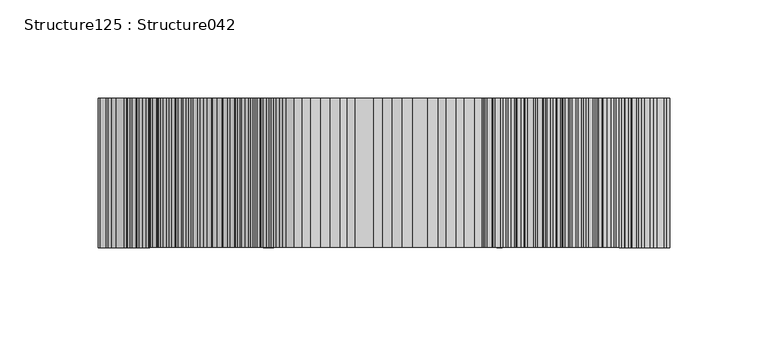
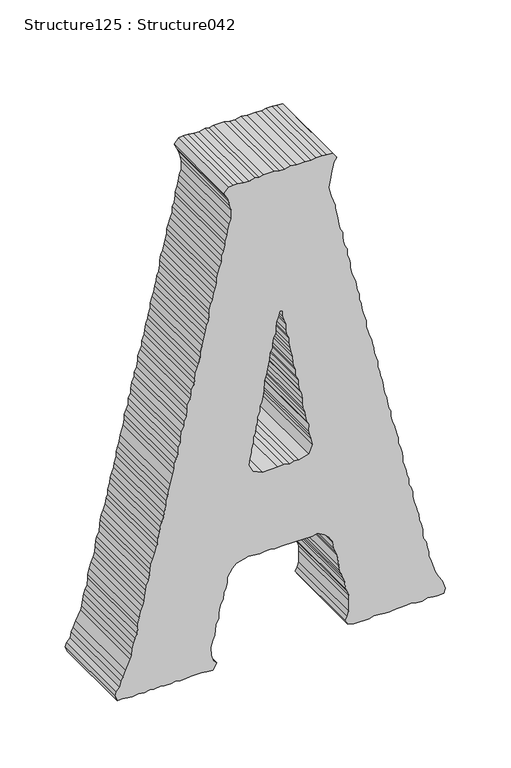
"""IFC4 building model written with IfcOpenShell, lengths in millimetres: proxy geometry, Structure125 : Structure042."""

from ifc_helpers import new_model, si_unit, frame, origin, place, context, project, spatial, polyline, outline, extrude, source, transform, mapped, element, save


def structure125_structure042_6af9a522(model_context):
    return source(origin(), model_context, "Body", "SweptSolid", [
        extrude(outline(polyline([(3818.8310229, -41243.193379), (3814.7296538, -41243.193379), (3811.2043377, -41244.3743679), (3805.9476534, -41246.6914168), (3801.8462843, -41246.6914168), (3795.960595, -41247.2931435), (3791.8865042, -41249.6326569), (3787.7867397, -41249.6326569), (3783.0868532, -41251.9962393), (3777.8285642, -41252.5755015), (3773.11905, -41252.5755015), (3769.6274306, -41254.9150149), (3763.759392, -41254.9150149), (3759.6596275, -41256.675266), (3755.559863, -41258.4371217), (3750.8583719, -41258.4371217), (3746.1745313, -41259.5956462), (3737.400554, -41261.9351595), (3732.1149867, -41263.1161484), (3727.4311462, -41264.2746729), (3723.3313817, -41265.4572664), (3718.6571688, -41265.4572664), (3713.3555556, -41267.2175175), (3709.2718371, -41267.8192442), (3704.5879966, -41269.5570309), (3701.0723082, -41270.7155553), (3695.786741, -41271.317282), (3690.512406, -41273.0791377), (3685.8285655, -41273.0791377), (3682.8857208, -41274.2601267), (3677.6274319, -41275.4186511), (3672.9435914, -41277.1789022), (3668.8261762, -41278.9391534), (3664.1423357, -41279.5184156), (3660.0682449, -41280.0992824), (3654.1841602, -41280.7010091), (3650.1004418, -41283.0405225), (3645.9830266, -41283.6422491), (3641.2991861, -41284.1990469), (3636.0408972, -41284.7783091), (3631.915459, -41285.959298), (3627.8397636, -41287.7211538), (3622.555801, -41289.4814049), (3617.2718384, -41290.6623938), (3613.772196, -41290.6623938), (3607.8961343, -41291.241656), (3604.3964919, -41293.0019072), (3600.2967274, -41294.1604316), (3595.5872132, -41295.3430251), (3589.7544759, -41295.9222873), (3586.2115092, -41297.1032763), (3577.4535778, -41301.2030407), (3572.1423369, -41303.5441587), (3568.6426945, -41305.3044098), (3563.366755, -41306.4629343), (3560.441561, -41309.4041743), (3556.3417965, -41310.5867678), (3551.6675836, -41308.8024476), (3551.6675836, -41304.1458854), (3551.0658569, -41299.4427896), (3550.4833855, -41295.3430251), (3551.6675836, -41290.0831316), (3550.4833855, -41284.7783091), (3551.6675836, -41280.0992824), (3551.0658569, -41276.5771755), (3551.6675836, -41270.7155553), (3551.0658569, -41267.2175175), (3551.0658569, -41261.3783618), (3551.6675836, -41257.2545282), (3551.0658569, -41253.1547637), (3551.0658569, -41248.4516679), (3551.6675836, -41243.7726412), (3551.6675836, -41234.4113786), (3551.0658569, -41229.7323519), (3550.4833855, -41224.4275294), (3556.3417965, -41220.9294916), (3559.2669905, -41223.8482672), (3565.1254015, -41225.6085183), (3572.7440636, -41226.1877806), (3578.6104977, -41224.4275294), (3582.7102621, -41222.6897428), (3587.3860796, -41222.1104805), (3592.0955938, -41221.5087539), (3596.7698067, -41219.1676359), (3601.4536473, -41219.1676359), (3604.9709403, -41218.5883737), (3610.2292293, -41217.4073848), (3613.772196, -41215.0678714), (3619.6145609, -41214.4886092), (3622.555801, -41212.7267535), (3627.8397636, -41211.5457645), (3633.0980525, -41211.5457645), (3639.5405396, -41206.8667378), (3643.0578326, -41203.344631), (3644.8245022, -41196.3244863), (3645.9830266, -41192.803984), (3645.4262289, -41186.9423638), (3644.8245022, -41182.8409947), (3645.4262289, -41178.161968), (3645.9830266, -41173.4588722), (3644.8245022, -41169.3815722), (3645.4262289, -41164.0767497), (3645.4262289, -41151.7967115), (3644.8245022, -41145.9350913), (3644.8245022, -41136.5529688), (3645.9830266, -41131.8739421), (3642.4833842, -41125.4330597), (3638.9580681, -41121.3092261), (3633.0980525, -41118.412915), (3627.2396415, -41117.2319261), (3622.555801, -41115.4700704), (3619.6145609, -41114.2890815), (3609.0723094, -41113.1080925), (3604.3964919, -41111.9271036), (3600.2967274, -41110.7910437), (3596.1953583, -41109.0291879), (3592.0955938, -41107.848199), (3586.2115092, -41107.2689368), (3582.7102621, -41105.4862212), (3578.6104977, -41104.3276967), (3573.9266571, -41104.3276967), (3563.9412034, -41104.3276967), (3559.2669905, -41105.4862212), (3555.7416744, -41107.2689368), (3551.6675836, -41104.906959), (3550.4833855, -41099.6470654), (3550.4833855, -41086.1635739), (3551.6675836, -41082.0638094), (3551.0658569, -41076.7814514), (3550.4833855, -41072.1024247), (3550.4833855, -41068.0010556), (3551.0658569, -41062.1394353), (3551.0658569, -41058.0621353), (3551.6675836, -41053.3590395), (3551.6675836, -41049.2576705), (3550.4833855, -41044.5561793), (3550.4833855, -41039.2962857), (3551.6675836, -41034.6156544), (3551.0658569, -41029.3124366), (3550.4833855, -41025.8127942), (3551.0658569, -41019.9736384), (3555.1848766, -41018.7926495), (3560.441561, -41020.5545052), (3563.366755, -41021.7130297), (3568.6426945, -41025.2335319), (3572.1423369, -41026.9937831), (3576.2693797, -41028.7556388), (3586.2115092, -41031.6744144), (3590.3289243, -41033.4346655), (3594.4286888, -41033.4346655), (3599.1125293, -41034.6156544), (3604.3964919, -41035.7757835), (3608.4705827, -41038.1152968), (3612.5976255, -41038.6945591), (3617.2718384, -41038.6945591), (3622.555801, -41039.875548), (3627.2396415, -41041.6357991), (3632.5155811, -41042.2375258), (3636.0408972, -41043.3976548), (3640.114988, -41044.5561793), (3645.4262289, -41046.3164304), (3650.6845178, -41047.4974193), (3655.3587307, -41047.4974193), (3659.4584952, -41048.6784082), (3663.5598643, -41051.0195262), (3668.8261762, -41051.0195262), (3673.5276674, -41052.7573129), (3677.0449605, -41053.3590395), (3682.8857208, -41055.1192907), (3686.4030139, -41056.2778151), (3691.0868544, -41056.2778151), (3695.2122926, -41056.8795418), (3699.8881101, -41058.0621353), (3705.7545441, -41060.3791842), (3710.4560353, -41060.3791842), (3714.5301261, -41061.5601731), (3718.0554422, -41062.7186976), (3723.3313817, -41063.8996865), (3727.4311462, -41065.6615422), (3732.7167134, -41066.8200667), (3737.9750024, -41066.8200667), (3740.9162424, -41068.5803178), (3745.6000829, -41069.7613067), (3751.4424479, -41070.3405689), (3756.1423345, -41072.1024247), (3759.6596275, -41073.2834136), (3764.3611187, -41073.8402113), (3769.0176809, -41074.441938), (3774.3032481, -41076.2021891), (3777.8285642, -41076.7814514), (3783.0868532, -41078.5417025), (3788.3611881, -41078.5417025), (3791.8865042, -41079.724296), (3797.1463977, -41081.4620827), (3801.8462843, -41082.0638094), (3806.5317294, -41083.2223338), (3810.0474179, -41083.8240605), (3815.3313805, -41086.1635739), (3820.015221, -41087.3461674), (3824.1149855, -41088.5271563), (3829.374879, -41088.5271563), (3837.6000817, -41091.4459319), (3842.8583706, -41092.6044563), (3846.9757858, -41093.206183), (3851.6612309, -41094.9680387), (3856.9179152, -41094.9680387), (3861.0192843, -41096.7058254), (3866.3032469, -41097.2850876), (3869.8189354, -41097.8868143), (3873.9203044, -41099.6470654), (3878.5784713, -41101.4073166), (3883.8881076, -41102.5899101), (3888.5623205, -41102.5899101), (3892.6636896, -41103.7484345), (3897.3475301, -41105.4862212), (3902.6314927, -41105.4862212), (3906.1487857, -41107.848199), (3910.8310217, -41109.0291879), (3916.0909152, -41109.6100547), (3919.6066036, -41109.6100547), (3924.2888396, -41111.9271036), (3928.9919353, -41113.1080925), (3934.2758979, -41113.7098192), (3938.9517154, -41114.8683437), (3944.235678, -41116.0493326), (3947.1496398, -41116.0493326), (3956.5349715, -41119.548975), (3961.794865, -41120.7299639), (3965.8930249, -41121.9109528), (3974.7055128, -41120.1507017), (3979.9621971, -41118.9697128), (3983.4794902, -41118.412915), (3987.5792547, -41117.2319261), (3991.6806238, -41114.8683437), (3996.390138, -41118.412915), (3996.9645864, -41123.6712039), (3997.5486624, -41127.7501086), (3997.5486624, -41133.054931), (3996.390138, -41137.1322311), (3996.9645864, -41142.4145891), (3996.9645864, -41150.0139959), (3997.5486624, -41155.3188184), (3996.390138, -41160.5771073), (3996.390138, -41165.2577387), (3997.5486624, -41169.9608344), (3997.5486624, -41179.3204925), (3996.9645864, -41183.4218615), (3997.5486624, -41186.9423638), (3996.390138, -41192.2247218), (3996.390138, -41196.9037485), (3997.5486624, -41202.1636421), (3997.5486624, -41206.2874756), (3996.9645864, -41210.3647756), (3992.2614906, -41214.4886092), (3987.5792547, -41212.1474912), (3984.0635662, -41210.3647756), (3979.3781211, -41209.2062512), (3974.7055128, -41208.0477267), (3966.5043792, -41208.0477267), (3962.3757319, -41209.7855134), (3957.1190475, -41210.9665023), (3952.435207, -41211.5457645), (3947.7337158, -41213.3076203), (3944.235678, -41213.3076203), (3938.3499888, -41214.4886092), (3934.8503464, -41216.2488603), (3929.5904528, -41216.2488603), (3924.8905662, -41217.986647), (3919.6066036, -41219.7468981), (3915.5068392, -41220.9294916), (3910.8310217, -41220.9294916), (3906.1487857, -41222.1104805), (3902.6314927, -41223.2914695), (3896.763454, -41224.4275294), (3893.822214, -41226.1877806), (3888.5623205, -41227.3687695), (3884.4609514, -41227.3687695), (3878.5784713, -41227.9704962), (3875.0772243, -41229.7323519), (3870.4030114, -41230.3116141), (3866.3032469, -41231.4701386), (3861.0192843, -41232.628663), (3856.9179152, -41233.8096519), (3851.6612309, -41235.5715077), (3846.9757858, -41235.5715077), (3841.6741725, -41237.3317588), (3838.1761347, -41237.9334855), (3833.4730389, -41239.6712721), (3828.2163546, -41240.2505344), (3824.1149855, -41240.8522611), (3818.8310229, -41243.193379)]), holes=[polyline([(3720.4158154, -41180.5014814), (3723.9154578, -41188.7026149), (3730.9323932, -41192.2247218), (3736.7988273, -41191.0437329), (3741.5003184, -41189.8836039), (3744.9999608, -41189.8836039), (3750.3015741, -41188.1008883), (3755.559863, -41188.1008883), (3759.0595054, -41186.3631016), (3764.3611187, -41185.7838394), (3768.4432325, -41184.6028505), (3773.11905, -41184.6028505), (3777.8285642, -41182.2617325), (3783.0868532, -41182.2617325), (3786.0280932, -41180.5014814), (3790.7039107, -41179.8997547), (3795.4037973, -41178.7636947), (3804.7730829, -41178.161968), (3810.0474179, -41176.4017169), (3814.7296538, -41175.8208501), (3818.8310229, -41174.6398611), (3822.932392, -41174.0605989), (3828.790803, -41173.4588722), (3833.4730389, -41171.1418233), (3836.9919366, -41171.1418233), (3842.2758992, -41170.5400967), (3845.8012153, -41168.1989787), (3851.0595042, -41168.1989787), (3855.7353217, -41167.6197165), (3860.4432313, -41165.8370009), (3865.1190488, -41164.6784764), (3864.5446004, -41162.9406898), (3860.4432313, -41162.9406898), (3856.3161885, -41161.7597009), (3851.6612309, -41159.9978451), (3846.3772683, -41159.9978451), (3842.2758992, -41159.3961184), (3837.6000817, -41157.0566051), (3832.8921721, -41157.0566051), (3828.790803, -41156.4773429), (3824.1149855, -41155.3188184), (3819.4150989, -41154.1378295), (3813.5743386, -41153.5569627), (3810.0474179, -41152.955236), (3805.9476534, -41151.1949849), (3800.6717138, -41151.1949849), (3795.4037973, -41148.8554715), (3790.7039107, -41148.8554715), (3786.0280932, -41147.6969471), (3782.5027771, -41145.9350913), (3777.2444882, -41145.3558291), (3772.5606477, -41145.3558291), (3767.8607611, -41144.7541024), (3763.759392, -41142.9938513), (3759.6596275, -41142.4145891), (3754.9854146, -41141.8128624), (3750.8583719, -41139.4958135), (3744.9999608, -41140.0750757), (3740.9162424, -41138.8940868), (3736.7988273, -41137.7339577), (3730.9323932, -41136.5529688), (3723.3313817, -41139.4958135), (3720.4158154, -41148.2762093), (3720.9726131, -41152.3759738), (3719.8140887, -41156.4773429), (3720.9726131, -41161.7597009), (3720.4158154, -41167.0179898), (3720.4158154, -41180.5014814)])]), frame((0.0, 247945.1599557, 0.0), z_axis=(0.0, 1.0, 0.0), x_axis=(0.0, 0.0, 1.0)), (0.0, 0.0, 1.0), 76.2),
    ])


if __name__ == "__main__":
    model = new_model("IFC4")
    model_context = context("Model", 3, world=origin())
    ifc_project = project(units=[si_unit("LENGTHUNIT", "METRE", prefix="MILLI")], contexts=[model_context])
    site = spatial("IfcSite", under=ifc_project)
    building = spatial("IfcBuilding", under=site)
    placement = place(None, origin())
    structure125_structure042_shape = structure125_structure042_6af9a522(model_context)
    element("IfcBuildingElementProxy", 1, Name="Structure125 : Structure042", ObjectType="Structure125 : Structure042", at=placement, inside=building, context=model_context, shape_type="MappedRepresentation", body=[
        mapped(structure125_structure042_shape, transform((0.0, 0.0, 0.0), x_axis=(1.0, 0.0, 0.0), y_axis=(0.0, 1.0, 0.0), z_axis=(0.0, 0.0, 1.0))),
    ])
    save(model, "model.ifc")

# Revit data of these elements
# Type "Structure125 : Structure042"
#   NameOverride = "Structure042"
# Element 1 (IfcBuildingElementProxy, "Structure125 : Structure042")
#   Materials on its faces: "BRUSHED ALUM. LETTERING"
# Materials
#   "BRUSHED ALUM. LETTERING": class "Unassigned", colour RGB 169 181 186, transparency 0, Cost = 0
